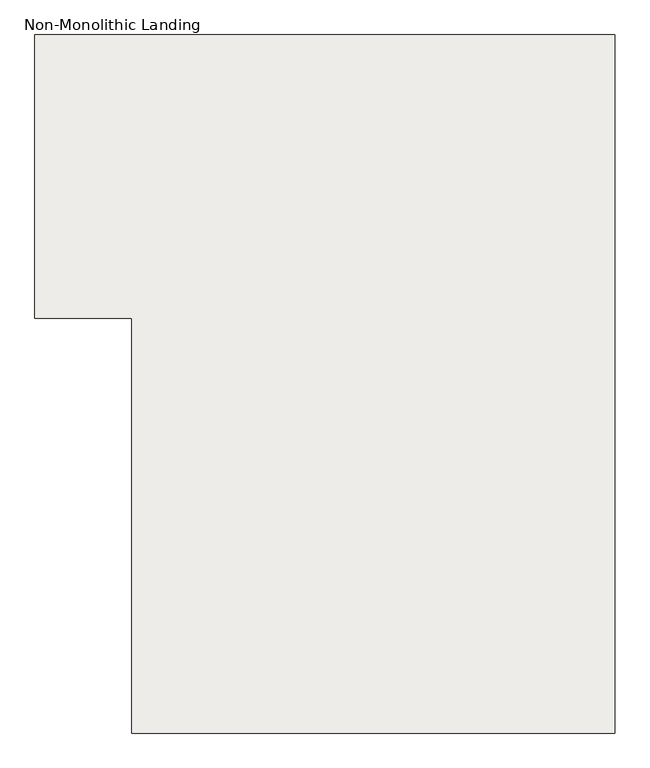
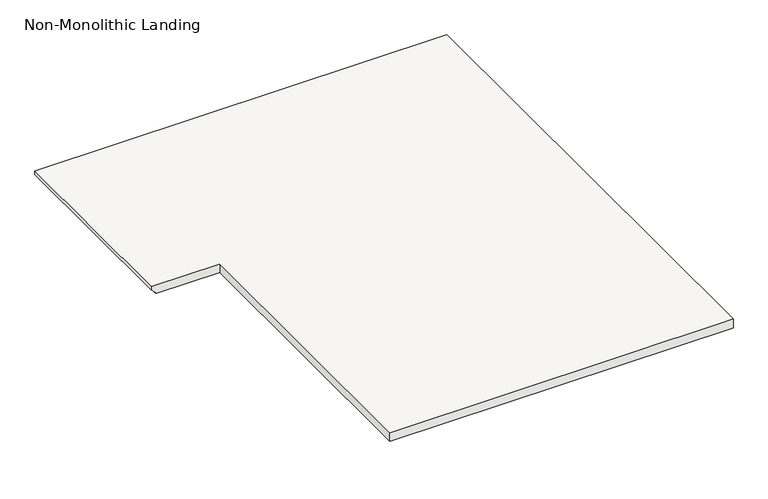
"""IFC4 building model written with IfcOpenShell, lengths in millimetres: slab geometry, Non-Monolithic Landing."""

import ifcopenshell
import ifcopenshell.guid

model = None  # the IFC model being written
_history = None  # IfcOwnerHistory: only IFC2X3 demands one
_inside = {}  # id of a spatial element -> (the spatial element, [elements in it])
_under = {}  # id of a project, library or spatial element -> (it, [spatial elements below it])
_declared = {}  # id of a project -> (the project, [libraries it declares])
_typed = {}  # id of a type object -> (the type object, [elements of that type])
_made_of = {}  # id of a material, layer set ... -> (it, [elements and type objects made of it])


def new_model(schema):
    """Start an empty IFC model of exactly this schema.

    Asked for "IFC4X3", IfcOpenShell would pick the latest addendum, in which some entities
    have other attributes; the version numbers below select the first issue.
    IFC2X3 requires an IfcOwnerHistory on every rooted entity: one is made here for all.
    """
    global model, _history
    if schema == "IFC4X3":
        model = ifcopenshell.file(schema_version=(4, 3, 0, 0))
    else:
        model = ifcopenshell.file(schema=schema)
    _inside.clear()
    _under.clear()
    _declared.clear()
    _typed.clear()
    _made_of.clear()
    _history = None
    if model.schema == "IFC2X3":
        org = make("IfcOrganization", Name="unknown")
        user = make(
            "IfcPersonAndOrganization",
            ThePerson=make("IfcPerson", FamilyName="unknown"),
            TheOrganization=org,
        )
        app = make(
            "IfcApplication",
            ApplicationDeveloper=org,
            Version="unknown",
            ApplicationFullName="unknown",
            ApplicationIdentifier="unknown",
        )
        _history = make(
            "IfcOwnerHistory",
            OwningUser=user,
            OwningApplication=app,
            ChangeAction="ADDED",
            CreationDate=0,
        )
    return model


def make(cls, **values):
    """One entity of the class cls with the attributes given. An attribute that is None is left unset."""
    return model.create_entity(
        cls, **{name: value for name, value in values.items() if value is not None}
    )


def rooted(cls, **values):
    """An entity with a GlobalId (a new one), such as an element, a storey or a relation."""
    return make(cls, GlobalId=ifcopenshell.guid.new(), OwnerHistory=_history, **values)


def si_unit(unit_type, name, prefix=None):
    """IfcSIUnit, for example si_unit("LENGTHUNIT", "METRE", prefix="MILLI")."""
    return make("IfcSIUnit", UnitType=unit_type, Prefix=prefix, Name=name)


def assignment(units):
    """IfcUnitAssignment: the units of a project."""
    return None if units is None else make("IfcUnitAssignment", Units=units)


def point(xyz):
    """IfcCartesianPoint."""
    return None if xyz is None else make("IfcCartesianPoint", Coordinates=xyz)


def direction(xyz):
    """IfcDirection."""
    return None if xyz is None else make("IfcDirection", DirectionRatios=xyz)


def frame(location, z_axis=None, x_axis=None):
    """IfcAxis2Placement3D, a coordinate frame: its origin and axes. An axis left out is left unset."""
    return make(
        "IfcAxis2Placement3D",
        Location=point(location),
        Axis=direction(z_axis),
        RefDirection=direction(x_axis),
    )


def origin():
    """The frame at (0, 0, 0) with its axes left unset."""
    return frame((0.0, 0.0, 0.0))


def place(relative_to, where):
    """IfcLocalPlacement: puts the frame where relative to a parent placement (None: the world)."""
    return make(
        "IfcLocalPlacement", PlacementRelTo=relative_to, RelativePlacement=where
    )


def context(
    kind, dimensions, precision=None, world=None, true_north=None, identifier=None
):
    """IfcGeometricRepresentationContext, for example the 3D "Model" context."""
    return make(
        "IfcGeometricRepresentationContext",
        ContextIdentifier=identifier,
        ContextType=kind,
        CoordinateSpaceDimension=dimensions,
        Precision=precision,
        WorldCoordinateSystem=world,
        TrueNorth=true_north,
    )


def project(units=None, contexts=None):
    """IfcProject with its units and contexts."""
    return rooted(
        "IfcProject",
        Name="project",
        RepresentationContexts=contexts,
        UnitsInContext=assignment(units),
    )


def spatial(cls, under=None, at=None, **own):
    """A site, building, storey or space (cls), placed at a placement, below another one or the project."""
    s = rooted(cls, ObjectPlacement=at, **own)
    if under is not None:
        _under.setdefault(under.id(), (under, []))[1].append(s)
    return s


def faces_of(points, faces, orient=None, outer=None):
    """IfcFace entities. A face is a list of loops; a loop is a list of indices into points, from 0.

    orient and outer hold one flag for each loop. By default every Orientation is true, the
    first loop of a face is its IfcFaceOuterBound and the others are IfcFaceBound.
    """
    made = []
    for i, loops in enumerate(faces):
        bounds = []
        for j, loop in enumerate(loops):
            is_outer = j == 0 if outer is None else outer[i][j]
            bounds.append(
                make(
                    "IfcFaceOuterBound" if is_outer else "IfcFaceBound",
                    Bound=make("IfcPolyLoop", Polygon=[points[k] for k in loop]),
                    Orientation=True if orient is None else orient[i][j],
                )
            )
        made.append(make("IfcFace", Bounds=bounds))
    return made


def faceted_brep(points, faces, orient=None, outer=None, voids=None):
    """IfcFacetedBrep: a solid bounded by flat faces; with voids (closed shells), ...WithVoids."""
    shared = [point(p) for p in points]
    hull = make("IfcClosedShell", CfsFaces=faces_of(shared, faces, orient, outer))
    if voids is None:
        return make("IfcFacetedBrep", Outer=hull)
    return make(
        "IfcFacetedBrepWithVoids",
        Outer=hull,
        Voids=[
            make(cls, CfsFaces=faces_of(shared, fs, o, b)) for cls, fs, o, b in voids
        ],
    )


def shape(context_of_items, identifier, shape_type, items):
    """IfcShapeRepresentation: the items that make up one representation, for example the "Body"."""
    return make(
        "IfcShapeRepresentation",
        ContextOfItems=context_of_items,
        RepresentationIdentifier=identifier,
        RepresentationType=shape_type,
        Items=items,
    )


def source(mapping_origin, context_of_items, identifier, shape_type, items):
    """IfcRepresentationMap: a shape defined once, which mapped items show again and again."""
    return make(
        "IfcRepresentationMap",
        MappingOrigin=mapping_origin,
        MappedRepresentation=shape(context_of_items, identifier, shape_type, items),
    )


def transform(
    local_origin,
    x_axis=None,
    y_axis=None,
    z_axis=None,
    scale=None,
    scale2=None,
    scale3=None,
    uniform=True,
):
    """IfcCartesianTransformationOperator3D, or its non-uniform kind. x_axis, y_axis, z_axis: its Axis1, 2, 3."""
    if uniform:
        return make(
            "IfcCartesianTransformationOperator3D",
            Axis1=direction(x_axis),
            Axis2=direction(y_axis),
            LocalOrigin=point(local_origin),
            Scale=scale,
            Axis3=direction(z_axis),
        )
    return make(
        "IfcCartesianTransformationOperator3DnonUniform",
        Axis1=direction(x_axis),
        Axis2=direction(y_axis),
        LocalOrigin=point(local_origin),
        Scale=scale,
        Axis3=direction(z_axis),
        Scale2=scale2,
        Scale3=scale3,
    )


def mapped(mapping_source, mapping_target):
    """IfcMappedItem: shows the shape of a source again, moved by a transform."""
    return make(
        "IfcMappedItem", MappingSource=mapping_source, MappingTarget=mapping_target
    )


def made_of(thing, what):
    """Note that an element or type object is made of a material, layer set ...; save() writes the relation."""
    if what is not None:
        _made_of.setdefault(what.id(), (what, []))[1].append(thing)
    return thing


def element(
    cls,
    number,
    at=None,
    inside=None,
    cuts=None,
    type_object=None,
    material=None,
    context=None,
    identifier="Body",
    shape_type=None,
    held_by="IfcProductDefinitionShape",
    body=None,
    shapes=None,
    **own,
):
    """One element of the class cls, such as IfcWall. Its Tag is "e" and its number.

    at: its placement. inside: the storey or other place that contains it. cuts: it is an
    opening in that element (IfcRelVoidsElement). A single representation is given by context,
    identifier, shape_type and body (its items); several are given by shapes. held_by: the class
    of the entity that holds the representations. save() writes the other relations.
    """
    e = rooted(cls, Tag="e%d" % number, ObjectPlacement=at, **own)
    if body is not None:
        shapes = [shape(context, identifier, shape_type, body)]
    if shapes is not None:
        e.Representation = make(held_by, Representations=shapes)
    if inside is not None:
        _inside.setdefault(inside.id(), (inside, []))[1].append(e)
    if cuts is not None:
        rooted(
            "IfcRelVoidsElement", RelatingBuildingElement=cuts, RelatedOpeningElement=e
        )
    if type_object is not None:
        _typed.setdefault(type_object.id(), (type_object, []))[1].append(e)
    return made_of(e, material)


def aggregate(whole, parts):
    """IfcRelAggregates: a whole, such as a stair, and the parts it consists of."""
    return rooted("IfcRelAggregates", RelatingObject=whole, RelatedObjects=parts)


def save(model, path):
    """Write the relations noted so far, then the file.

    IfcRelAggregates (storeys below a building ...), IfcRelContainedInSpatialStructure (elements
    in a storey), IfcRelDefinesByType, IfcRelAssociatesMaterial and IfcRelDeclares: one each for
    every whole, place, type object, material and project.
    """
    for whole, parts in _under.values():
        aggregate(whole, parts)
    for where, things in _inside.values():
        rooted(
            "IfcRelContainedInSpatialStructure",
            RelatedElements=things,
            RelatingStructure=where,
        )
    for kind, things in _typed.values():
        rooted("IfcRelDefinesByType", RelatedObjects=things, RelatingType=kind)
    for what, things in _made_of.values():
        rooted("IfcRelAssociatesMaterial", RelatedObjects=things, RelatingMaterial=what)
    for by, libraries in _declared.values():
        rooted("IfcRelDeclares", RelatingContext=by, RelatedDefinitions=libraries)
    model.write(path)


def non_monolithic_landing_a3dac32d(model_context):
    return source(origin(), model_context, "Body", "Brep", [
        faceted_brep([(-937.2122732, 8132.6265304, 0.0), (-937.2122732, 6497.5015304, 0.0), (967.7877268, 6497.5015304, 0.0), (967.7877268, 9250.2265304, 0.0), (-1318.2122732, 9250.2265304, 0.0), (-1318.2122732, 8132.6265304, 0.0), (-1292.8122732, 8132.6265304, -50.8), (-1292.8122732, 9250.2265304, -50.8), (967.7877268, 9250.2265304, -50.8), (967.7877268, 6497.5015304, -50.8), (-937.2122732, 6497.5015304, -50.8), (-937.2122732, 8132.6265304, -50.8), (-1292.8122732, 9250.2265304, -44.45), (-1318.2122732, 9250.2265304, -19.05), (-1318.2122732, 8132.6265304, -19.05), (-1292.8122732, 8132.6265304, -44.45)], [[[0, 1, 2, 3, 4, 5]], [[6, 7, 8, 9, 10, 11]], [[1, 0, 11, 10]], [[2, 1, 10, 9]], [[3, 2, 9, 8]], [[4, 3, 8, 7, 12, 13]], [[0, 5, 14, 15, 6, 11]], [[7, 6, 15, 12]], [[14, 5, 4, 13]], [[15, 14, 13, 12]]]),
    ])


if __name__ == "__main__":
    model = new_model("IFC4")
    model_context = context("Model", 3, world=origin())
    ifc_project = project(units=[si_unit("LENGTHUNIT", "METRE", prefix="MILLI")], contexts=[model_context])
    site = spatial("IfcSite", under=ifc_project)
    building = spatial("IfcBuilding", under=site)
    placement = place(None, origin())
    non_monolithic_landing_shape = non_monolithic_landing_a3dac32d(model_context)
    element("IfcSlab", 1, ObjectType="Non-Monolithic Landing", at=placement, inside=building, context=model_context, shape_type="MappedRepresentation", body=[
        mapped(non_monolithic_landing_shape, transform((0.0, 0.0, 0.0), x_axis=(1.0, 0.0, 0.0), y_axis=(0.0, 1.0, 0.0), z_axis=(0.0, 0.0, 1.0))),
    ])
    save(model, "model.ifc")
